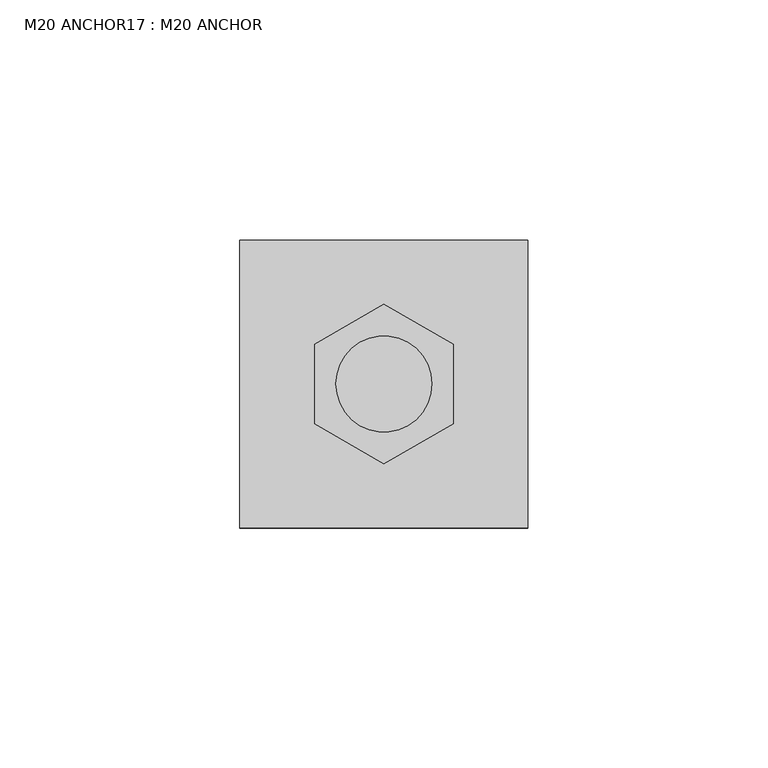
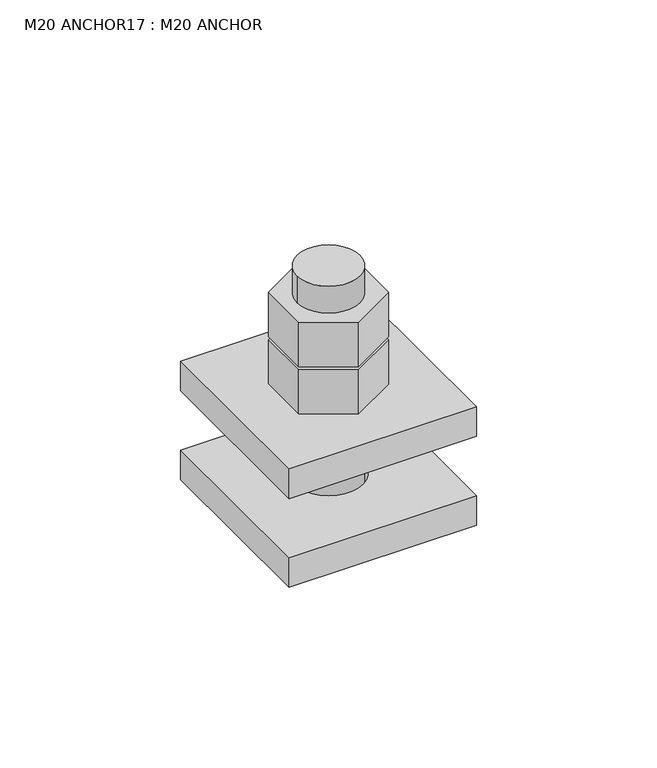
"""IFC4 building model written with IfcOpenShell, lengths in millimetres: fastener geometry, M20 ANCHOR17 : M20 ANCHOR."""

from ifc_helpers import new_model, si_unit, point, frame, frame_2d, origin, place, context, project, spatial, polyline, circle_curve, trimmed, segment, composite_curve, outline, extrude, source, transform, mapped, element, save


def m20_anchor17_m20_anchor_2c01de18(model_context):
    return source(origin(), model_context, "Body", "SweptSolid", [
        extrude(outline(polyline([(-8.0855968, 22545.0952779), (-8.0855968, 22528.4582151), (-22.4937158, 22520.1396837), (-36.9018348, 22528.4582151), (-36.9018348, 22545.0952779), (-22.4937158, 22553.4138093), (-8.0855968, 22545.0952779)]), holes=[composite_curve([segment(trimmed(circle_curve(frame_2d((-22.4937158, 22536.7767465)), 10.0), [point((-32.4937158, 22536.7767465))], [point((-12.4937158, 22536.7767465))], True, "CARTESIAN"), True, "CONTINUOUS"), segment(trimmed(circle_curve(frame_2d((-22.4937158, 22536.7767465)), 10.0), [point((-12.4937158, 22536.7767465))], [point((-32.4937158, 22536.7767465))], True, "CARTESIAN"), True, "CONTINUOUS")], self_intersect=False)]), frame((0.0, 0.0, 246.0), z_axis=(0.0, 0.0, 1.0), x_axis=(1.0, 0.0, 0.0)), (0.0, 0.0, 1.0), 15.0),
        extrude(outline(polyline([(-8.0855968, 22545.0952779), (-8.0855968, 22528.4582151), (-22.4937158, 22520.1396837), (-36.9018348, 22528.4582151), (-36.9018348, 22545.0952779), (-22.4937158, 22553.4138093), (-8.0855968, 22545.0952779)]), holes=[composite_curve([segment(trimmed(circle_curve(frame_2d((-22.4937158, 22536.7767465)), 10.0), [point((-32.4937158, 22536.7767465))], [point((-12.4937158, 22536.7767465))], True, "CARTESIAN"), True, "CONTINUOUS"), segment(trimmed(circle_curve(frame_2d((-22.4937158, 22536.7767465)), 10.0), [point((-12.4937158, 22536.7767465))], [point((-32.4937158, 22536.7767465))], True, "CARTESIAN"), True, "CONTINUOUS")], self_intersect=False)]), frame((0.0, 0.0, 230.0), z_axis=(0.0, 0.0, 1.0), x_axis=(1.0, 0.0, 0.0)), (0.0, 0.0, 1.0), 15.0),
        extrude(outline(composite_curve([segment(trimmed(circle_curve(frame_2d((-22.4937158, 22536.7767465)), 10.0), [point((-32.4937158, 22536.7767465))], [point((-12.4937158, 22536.7767465))], False, "CARTESIAN"), True, "CONTINUOUS"), segment(trimmed(circle_curve(frame_2d((-22.4937158, 22536.7767465)), 10.0), [point((-12.4937158, 22536.7767465))], [point((-32.4937158, 22536.7767465))], False, "CARTESIAN"), True, "CONTINUOUS")], self_intersect=False)), frame((0.0, 0.0, 190.0), z_axis=(0.0, 0.0, 1.0), x_axis=(1.0, 0.0, 0.0)), (0.0, 0.0, 1.0), 80.0),
        extrude(outline(polyline([(7.5062842, 22566.7767465), (7.5062842, 22506.7767465), (-52.4937158, 22506.7767465), (-52.4937158, 22566.7767465), (7.5062842, 22566.7767465)]), holes=[composite_curve([segment(trimmed(circle_curve(frame_2d((-22.4937158, 22536.7767465)), 11.0), [point((-33.4937158, 22536.7767465))], [point((-11.4937158, 22536.7767465))], True, "CARTESIAN"), True, "CONTINUOUS"), segment(trimmed(circle_curve(frame_2d((-22.4937158, 22536.7767465)), 11.0), [point((-11.4937158, 22536.7767465))], [point((-33.4937158, 22536.7767465))], True, "CARTESIAN"), True, "CONTINUOUS")], self_intersect=False)]), frame((0.0, 0.0, 190.0), z_axis=(0.0, 0.0, 1.0), x_axis=(1.0, 0.0, 0.0)), (0.0, 0.0, 1.0), 10.0),
        extrude(outline(polyline([(7.5062842, 22566.7767465), (7.5062842, 22506.7767465), (-52.4937158, 22506.7767465), (-52.4937158, 22566.7767465), (7.5062842, 22566.7767465)]), holes=[composite_curve([segment(trimmed(circle_curve(frame_2d((-22.4937158, 22536.7767465)), 11.0), [point((-33.4937158, 22536.7767465))], [point((-11.4937158, 22536.7767465))], True, "CARTESIAN"), True, "CONTINUOUS"), segment(trimmed(circle_curve(frame_2d((-22.4937158, 22536.7767465)), 11.0), [point((-11.4937158, 22536.7767465))], [point((-33.4937158, 22536.7767465))], True, "CARTESIAN"), True, "CONTINUOUS")], self_intersect=False)]), frame((0.0, 0.0, 220.0), z_axis=(0.0, 0.0, 1.0), x_axis=(1.0, 0.0, 0.0)), (0.0, 0.0, 1.0), 10.0),
    ])


if __name__ == "__main__":
    model = new_model("IFC4")
    model_context = context("Model", 3, world=origin())
    ifc_project = project(units=[si_unit("LENGTHUNIT", "METRE", prefix="MILLI")], contexts=[model_context])
    site = spatial("IfcSite", under=ifc_project)
    building = spatial("IfcBuilding", under=site)
    placement = place(None, origin())
    m20_anchor17_m20_anchor_shape = m20_anchor17_m20_anchor_2c01de18(model_context)
    element("IfcFastener", 1, ObjectType="M20 ANCHOR17 : M20 ANCHOR", at=placement, inside=building, context=model_context, shape_type="MappedRepresentation", body=[
        mapped(m20_anchor17_m20_anchor_shape, transform((0.0, 0.0, 0.0), x_axis=(1.0, 0.0, 0.0), y_axis=(0.0, 1.0, 0.0), z_axis=(0.0, 0.0, 1.0))),
    ])
    save(model, "model.ifc")
